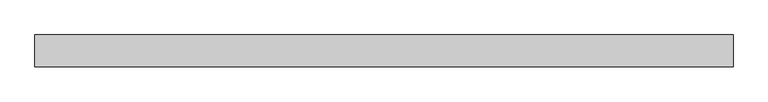
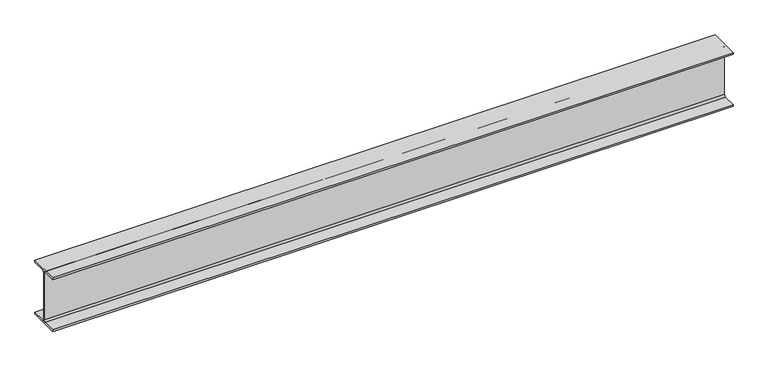
"""IFC4 building model written with IfcOpenShell, lengths in millimetres: beam geometry, Old_Steel Beam_H-KSD3502 : H_SB_ASB_H-200×200x8x12."""

from ifc_helpers import new_model, si_unit, point, frame, frame_2d, origin, place, context, project, spatial, polyline, circle_curve, trimmed, segment, composite_curve, outline, extrude, source, transform, mapped, element, save


def beam_c6904957(model_context):
    return source(origin(), model_context, "Body", "SweptSolid", [
        extrude(outline(composite_curve([segment(polyline([(82.5, -141.5), (82.5, -151.7), (-82.5, -151.7), (-82.5, -141.5), (-11.9, -141.5)]), True, "CONTINUOUS"), segment(trimmed(circle_curve(frame_2d((-11.9, -132.6)), 8.9), [point((-11.9, -141.5))], [point((-3.0, -132.6))], True, "CARTESIAN"), True, "CONTINUOUS"), segment(polyline([(-3.0, -132.6), (-3.0, 132.6)]), True, "CONTINUOUS"), segment(trimmed(circle_curve(frame_2d((-11.9, 132.6)), 8.9), [point((-3.0, 132.6))], [point((-11.9, 141.5))], True, "CARTESIAN"), True, "CONTINUOUS"), segment(polyline([(-11.9, 141.5), (-82.5, 141.5), (-82.5, 151.7), (82.5, 151.7), (82.5, 141.5), (11.9, 141.5)]), True, "CONTINUOUS"), segment(trimmed(circle_curve(frame_2d((11.9, 132.6)), 8.9), [point((11.9, 141.5))], [point((3.0, 132.6))], True, "CARTESIAN"), True, "CONTINUOUS"), segment(polyline([(3.0, 132.6), (3.0, -132.6)]), True, "CONTINUOUS"), segment(trimmed(circle_curve(frame_2d((11.9, -132.6)), 8.9), [point((3.0, -132.6))], [point((11.9, -141.5))], True, "CARTESIAN"), True, "CONTINUOUS"), segment(polyline([(11.9, -141.5), (82.5, -141.5)]), True, "CONTINUOUS")], self_intersect=False)), frame((-1780.1436483, 0.0, 0.0), z_axis=(1.0, 0.0, 0.0), x_axis=(0.0, 1.0, 0.0)), (0.0, 0.0, 1.0), 3630.9979746),
    ])


if __name__ == "__main__":
    model = new_model("IFC4")
    model_context = context("Model", 3, world=origin())
    ifc_project = project(units=[si_unit("LENGTHUNIT", "METRE", prefix="MILLI")], contexts=[model_context])
    site = spatial("IfcSite", under=ifc_project)
    building = spatial("IfcBuilding", under=site)
    placement = place(None, origin())
    beam_shape = beam_c6904957(model_context)
    element("IfcBeam", 1, ObjectType="Old_Steel Beam_H-KSD3502 : H_SB_ASB_H-200×200x8x12", at=placement, inside=building, context=model_context, shape_type="MappedRepresentation", body=[
        mapped(beam_shape, transform((0.0, 0.0, 0.0), x_axis=(1.0, 0.0, 0.0), y_axis=(0.0, 1.0, 0.0), z_axis=(0.0, 0.0, 1.0))),
    ])
    save(model, "model.ifc")

# Revit data of these elements
# Type "Old_Steel Beam_H-KSD3502 : H_SB_ASB_H-200×200x8x12"
#   Width = 20.0 cm
#   Web Thickness = 0.8 cm
#   Web Fillet = 1.3 cm
#   Warping Constant = 141376.0 cm⁶
#   Torsional Moment of Inertia = 26.2485 cm⁴
#   Torsional Modulus = 1.0 cm³
#   Section Area = 63.53 cm²
#   Plastic Modulus weak axis = 244.0 cm³
#   Plastic Modulus strong axis = 525.0 cm³
#   Perimeter = 1.16 m²/m
#   Nominal Weight = 49.90 kgf/m
#   Moment of Inertia weak axis = 1600.00 cm⁴
#   Moment of Inertia strong axis = 4720.00 cm⁴
#   Height = 20.0 cm
#   Flange Thickness = 1.2 cm
#   Elastic Modulus weak axis = 160.0 cm³
#   Elastic Modulus strong axis = 472.0 cm³
#   Centroid Vertical = 10.0 cm
#   Centroid Horizontal = 10.0 cm
#   Length [instance default] = 1.5240 m
#   Structural Material [instance default] = Steel, 45-345
#   Assembly Code = ""
# Element 1 (IfcBeam, "Old_Steel Beam_H-KSD3502 : H_SB_ASB_H-200×200x8x12")
#   Structural Material = none
# Materials
#   "Steel, 45-345": class "Metal", colour RGB 189 187 185, transparency 0, Description = "Steel 345 MPa", Cost = 0
